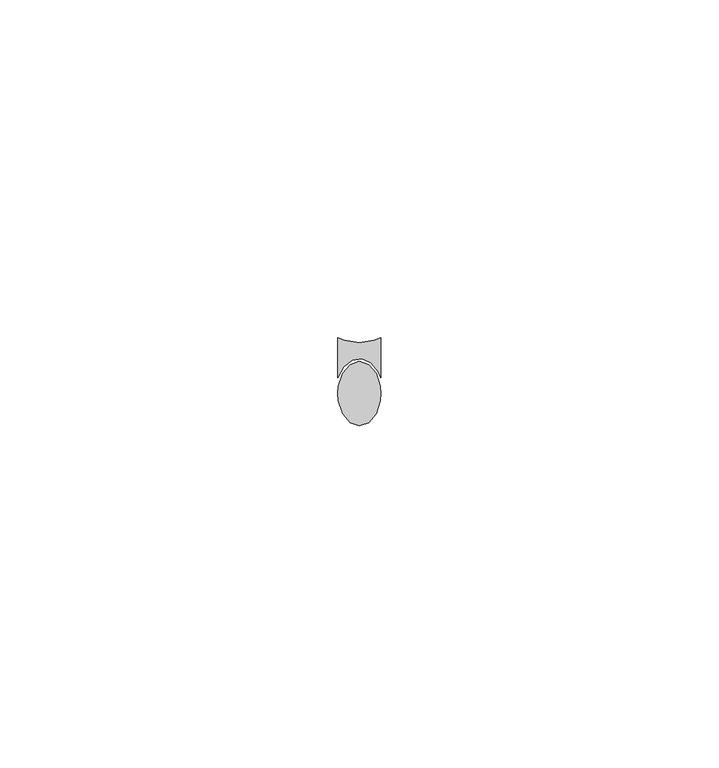
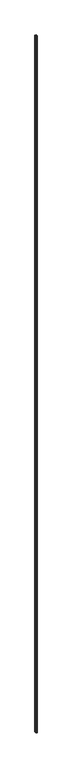
"""IFC4 building model written with IfcOpenShell, lengths in millimetres: proxy geometry, Generic Models 11:Generic Models 1:306267:Generic Models 1:306267 : Generic Models 11:Generic Models 1:306267:300405:Generic Models 1:306267:Generic Models 1:306267 : Generic Models 11:Generic Models 1:306267:300405 : Generic Models 11:Generic Models 1:306267:Generic Models 1:306267 : Generic Models 11:Generic Models 1:306267:300405:25 : Generic Models 11:Generic Models 1:306267:Generic Models 1:306267 : Generic Models 11:Generic Models 1:306267:300405:Generic Models 1:306267:Generic Models 1:306267 : Generic Models 11:Generic Models 1:306267:300405 : Generic Models 11:Generic Models 1:306267:Generic Models 1:306267 : Generic Models 11:Generic Models 1:306267:300405:300182."""

from ifc_helpers import new_model, si_unit, frame, origin, place, context, project, spatial, polyline, outline, extrude, source, transform, mapped, element, save


def generic_models_47283755(model_context):
    return source(origin(), model_context, "Body", "SweptSolid", [
        extrude(outline(polyline([(594928.7897638, -579036.3403513), (594929.8944979, -579037.6618453), (594930.507579, -579039.5714595), (594930.5871829, -579040.6312155), (594930.507579, -579041.6909714), (594929.8944979, -579043.6005857), (594928.7897638, -579044.9220797), (594927.4121829, -579045.3937155), (594926.034602, -579044.9220797), (594924.929868, -579043.6005857), (594924.3167868, -579041.6909714), (594924.2371829, -579040.6312155), (594924.3167868, -579039.5714595), (594924.929868, -579037.6618453), (594926.034602, -579036.3403513), (594927.4121829, -579035.8687155), (594928.7897638, -579036.3403513)])), frame((0.0, 0.0, 31.75), z_axis=(0.0, 0.0, 1.0), x_axis=(1.0, 0.0, 0.0)), (0.0, 0.0, 1.0), 3663.95),
        extrude(outline(polyline([(594925.2029461, -579032.7769044), (594927.4121829, -579033.0905905), (594929.6214197, -579032.7769044), (594930.5871829, -579032.3994958), (594930.5871829, -579038.2675879), (594930.2008653, -579037.4073069), (594929.1173799, -579036.0977318), (594927.7671321, -579035.4973783), (594926.3613558, -579035.7001662), (594925.1199717, -579036.6743712), (594924.2371829, -579038.2675879), (594924.2371829, -579032.3994958), (594925.2029461, -579032.7769044)])), frame((0.0, 0.0, 31.75), z_axis=(0.0, 0.0, 1.0), x_axis=(1.0, 0.0, 0.0)), (0.0, 0.0, 1.0), 3663.95),
    ])


if __name__ == "__main__":
    model = new_model("IFC4")
    model_context = context("Model", 3, world=origin())
    ifc_project = project(units=[si_unit("LENGTHUNIT", "METRE", prefix="MILLI")], contexts=[model_context])
    site = spatial("IfcSite", under=ifc_project)
    building = spatial("IfcBuilding", under=site)
    placement = place(None, origin())
    generic_models_shape = generic_models_47283755(model_context)
    element("IfcBuildingElementProxy", 1, Name="Generic Models 11:Generic Models 1:306267:Generic Models 1:306267 : Generic Models 11:Generic Models 1:306267:300405:Generic Models 1:306267:Generic Models 1:306267 : Generic Models 11:Generic Models 1:306267:300405 : Generic Models 11:Generic Models 1:306267:Generic Models 1:306267 : Generic Models 11:Generic Models 1:306267:300405:25 : Generic Models 11:Generic Models 1:306267:Generic Models 1:306267 : Generic Models 11:Generic Models 1:306267:300405:Generic Models 1:306267:Generic Models 1:306267 : Generic Models 11:Generic Models 1:306267:300405 : Generic Models 11:Generic Models 1:306267:Generic Models 1:306267 : Generic Models 11:Generic Models 1:306267:300405:300182", ObjectType="Generic Models 11:Generic Models 1:306267:Generic Models 1:306267 : Generic Models 11:Generic Models 1:306267:300405:Generic Models 1:306267:Generic Models 1:306267 : Generic Models 11:Generic Models 1:306267:300405 : Generic Models 11:Generic Models 1:306267:Generic Models 1:306267 : Generic Models 11:Generic Models 1:306267:300405:25 : Generic Models 11:Generic Models 1:306267:Generic Models 1:306267 : Generic Models 11:Generic Models 1:306267:300405:Generic Models 1:306267:Generic Models 1:306267 : Generic Models 11:Generic Models 1:306267:300405 : Generic Models 11:Generic Models 1:306267:Generic Models 1:306267 : Generic Models 11:Generic Models 1:306267:300405:300182", at=placement, inside=building, context=model_context, shape_type="MappedRepresentation", body=[
        mapped(generic_models_shape, transform((0.0, 0.0, 0.0), x_axis=(1.0, 0.0, 0.0), y_axis=(0.0, 1.0, 0.0), z_axis=(0.0, 0.0, 1.0))),
    ])
    save(model, "model.ifc")

# Revit data of these elements
# Type "Generic Models 11:Generic Models 1:306267:Generic Models 1:306267 : Generic Models 11:Generic Models 1:306267:300405:Generic Models 1:306267:Generic Models 1:306267 : Generic Models 11:Generic Models 1:306267:300405 : Generic Models 11:Generic Models 1:306267:Generic Models 1:306267 : Generic Models 11:Generic Models 1:306267:300405:25 : Generic Models 11:Generic Models 1:306267:Generic Models 1:306267 : Generic Models 11:Generic Models 1:306267:300405:Generic Models 1:306267:Generic Models 1:306267 : Generic Models 11:Generic Models 1:306267:300405 : Generic Models 11:Generic Models 1:306267:Generic Models 1:306267 : Generic Models 11:Generic Models 1:306267:300405:300182"
#   NameOverride = "Generic Models 11:Generic Models 1:306267:Generic Models 1:306267 : Generic Models 11:Generic Models 1:306267:300405:Generic Models 1:306267:Generic Models 1:306267 : Generic Models 11:Generic Models 1:306267:300405 : Generic Models 11:Generic Models 1:306267:Generic Models 1:306267 : Generic Models 11:Generic Models 1:306267:300405:300182"
#   ObjectTypeOverride = "Generic Models 1:306267:Generic Models 1:306267 : Generic Models 11:Generic Models 1:306267:300405 : Generic Models 11:Generic Models 1:306267:Generic Models 1:306267 : Generic Models 11:Generic Models 1:306267:300405"
#   Reference = "Generic Models 1"
#   Tag = "300182"
# Element 1 (IfcBuildingElementProxy, "Generic Models 11:Generic Models 1:306267:Generic Models 1:306267 : Generic Models 11:Generic Models 1:306267:300405:Generic Models 1:306267:Generic Models 1:306267 : Generic Models 11:Generic Models 1:306267:300405 : Generic Models 11:Generic Models 1:306267:Generic Models 1:306267 : Generic Models 11:Generic Models 1:306267:300405:25 : Generic Models 11:Generic Models 1:306267:Generic Models 1:306267 : Generic Models 11:Generic Models 1:306267:300405:Generic Models 1:306267:Generic Models 1:306267 : Generic Models 11:Generic Models 1:306267:300405 : Generic Models 11:Generic Models 1:306267:Generic Models 1:306267 : Generic Models 11:Generic Models 1:306267:300405:300182")
#   Materials on its faces: "SEALANT & BACKER ROD, IF NECESSARY"
# Materials
#   "SEALANT & BACKER ROD, IF NECESSARY": class "Unassigned", colour RGB 120 120 120, transparency 0, Cost = 0
